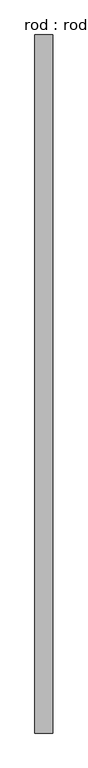
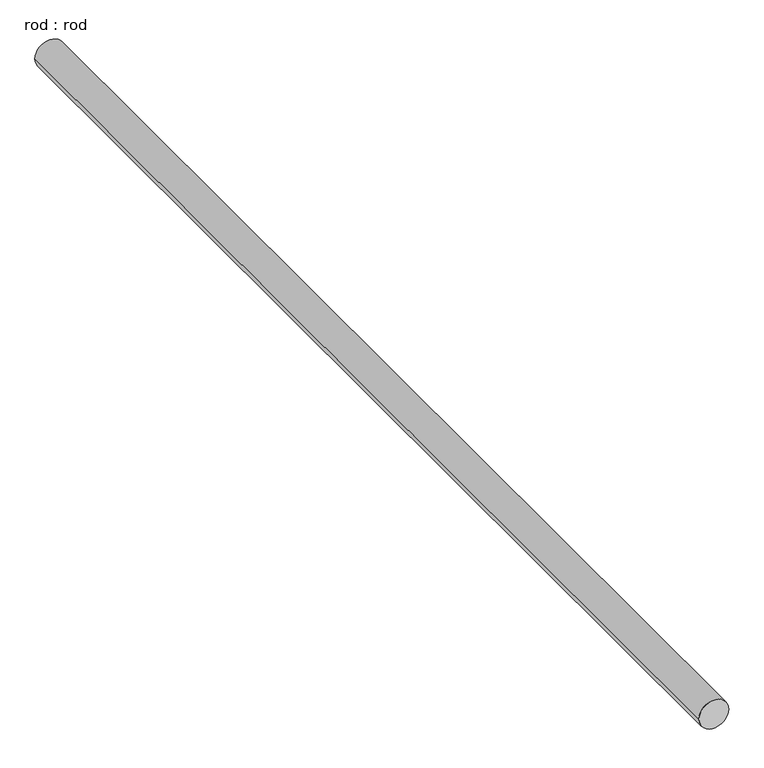
"""IFC4 building model written with IfcOpenShell, lengths in millimetres: proxy geometry, rod : rod."""

from ifc_helpers import new_model, si_unit, point, frame, frame_2d, origin, place, context, project, spatial, circle_curve, trimmed, segment, composite_curve, outline, extrude, source, transform, mapped, element, save


def rod_rod_39af1a0a(model_context):
    return source(origin(), model_context, "Body", "SweptSolid", [
        extrude(outline(composite_curve([segment(trimmed(circle_curve(frame_2d((0.0108462, 0.0)), 200.0), [point((0.0108462, 200.0))], [point((0.0108462, -200.0))], False, "CARTESIAN"), True, "CONTINUOUS"), segment(trimmed(circle_curve(frame_2d((0.0108462, 0.0)), 200.0), [point((0.0108462, -200.0))], [point((0.0108462, 200.0))], False, "CARTESIAN"), True, "CONTINUOUS")], self_intersect=False)), frame((0.0, -3650.2234218, 0.0), z_axis=(0.0, 1.0, 0.0), x_axis=(0.0, 0.0, 1.0)), (0.0, 0.0, 1.0), 15485.9040744),
    ])


if __name__ == "__main__":
    model = new_model("IFC4")
    model_context = context("Model", 3, world=origin())
    ifc_project = project(units=[si_unit("LENGTHUNIT", "METRE", prefix="MILLI")], contexts=[model_context])
    site = spatial("IfcSite", under=ifc_project)
    building = spatial("IfcBuilding", under=site)
    placement = place(None, origin())
    rod_rod_shape = rod_rod_39af1a0a(model_context)
    element("IfcBuildingElementProxy", 1, Name="rod : rod", ObjectType="rod : rod", at=placement, inside=building, context=model_context, shape_type="MappedRepresentation", body=[
        mapped(rod_rod_shape, transform((0.0, 0.0, 0.0), x_axis=(1.0, 0.0, 0.0), y_axis=(0.0, 1.0, 0.0), z_axis=(0.0, 0.0, 1.0))),
    ])
    save(model, "model.ifc")

# Revit data of these elements
# Type "rod : rod"
#   Default Elevation = 0
